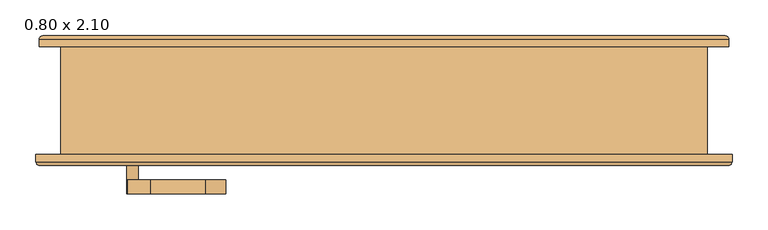
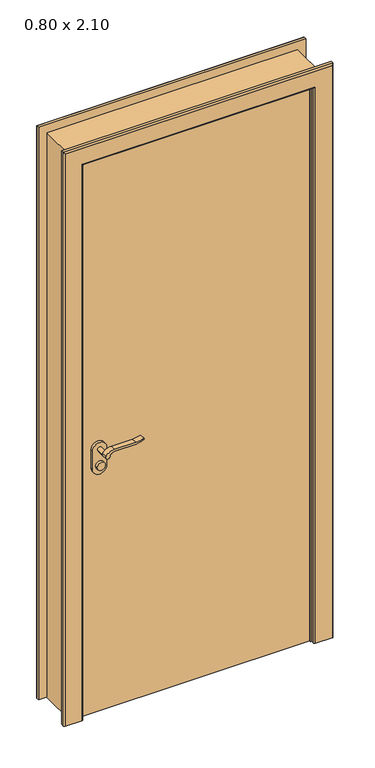
"""IFC4 building model written with IfcOpenShell, lengths in millimetres: door geometry, PORTA_DE_ABRIR_MADEIRA : 0.80 x 2.10."""

import ifcopenshell
import ifcopenshell.guid

model = None  # the IFC model being written
_history = None  # IfcOwnerHistory: only IFC2X3 demands one
_inside = {}  # id of a spatial element -> (the spatial element, [elements in it])
_under = {}  # id of a project, library or spatial element -> (it, [spatial elements below it])
_declared = {}  # id of a project -> (the project, [libraries it declares])
_typed = {}  # id of a type object -> (the type object, [elements of that type])
_made_of = {}  # id of a material, layer set ... -> (it, [elements and type objects made of it])


def new_model(schema):
    """Start an empty IFC model of exactly this schema.

    Asked for "IFC4X3", IfcOpenShell would pick the latest addendum, in which some entities
    have other attributes; the version numbers below select the first issue.
    IFC2X3 requires an IfcOwnerHistory on every rooted entity: one is made here for all.
    """
    global model, _history
    if schema == "IFC4X3":
        model = ifcopenshell.file(schema_version=(4, 3, 0, 0))
    else:
        model = ifcopenshell.file(schema=schema)
    _inside.clear()
    _under.clear()
    _declared.clear()
    _typed.clear()
    _made_of.clear()
    _history = None
    if model.schema == "IFC2X3":
        org = make("IfcOrganization", Name="unknown")
        user = make(
            "IfcPersonAndOrganization",
            ThePerson=make("IfcPerson", FamilyName="unknown"),
            TheOrganization=org,
        )
        app = make(
            "IfcApplication",
            ApplicationDeveloper=org,
            Version="unknown",
            ApplicationFullName="unknown",
            ApplicationIdentifier="unknown",
        )
        _history = make(
            "IfcOwnerHistory",
            OwningUser=user,
            OwningApplication=app,
            ChangeAction="ADDED",
            CreationDate=0,
        )
    return model


def make(cls, **values):
    """One entity of the class cls with the attributes given. An attribute that is None is left unset."""
    return model.create_entity(
        cls, **{name: value for name, value in values.items() if value is not None}
    )


def rooted(cls, **values):
    """An entity with a GlobalId (a new one), such as an element, a storey or a relation."""
    return make(cls, GlobalId=ifcopenshell.guid.new(), OwnerHistory=_history, **values)


def si_unit(unit_type, name, prefix=None):
    """IfcSIUnit, for example si_unit("LENGTHUNIT", "METRE", prefix="MILLI")."""
    return make("IfcSIUnit", UnitType=unit_type, Prefix=prefix, Name=name)


def assignment(units):
    """IfcUnitAssignment: the units of a project."""
    return None if units is None else make("IfcUnitAssignment", Units=units)


def point(xyz):
    """IfcCartesianPoint."""
    return None if xyz is None else make("IfcCartesianPoint", Coordinates=xyz)


def direction(xyz):
    """IfcDirection."""
    return None if xyz is None else make("IfcDirection", DirectionRatios=xyz)


def frame(location, z_axis=None, x_axis=None):
    """IfcAxis2Placement3D, a coordinate frame: its origin and axes. An axis left out is left unset."""
    return make(
        "IfcAxis2Placement3D",
        Location=point(location),
        Axis=direction(z_axis),
        RefDirection=direction(x_axis),
    )


def frame_2d(location, x_axis=None):
    """IfcAxis2Placement2D, a coordinate frame in the plane: its origin and x axis."""
    return make(
        "IfcAxis2Placement2D", Location=point(location), RefDirection=direction(x_axis)
    )


def origin():
    """The frame at (0, 0, 0) with its axes left unset."""
    return frame((0.0, 0.0, 0.0))


def origin_with_axes():
    """The frame at (0, 0, 0) with the z axis (0, 0, 1) and the x axis (1, 0, 0) written out."""
    return frame((0.0, 0.0, 0.0), z_axis=(0.0, 0.0, 1.0), x_axis=(1.0, 0.0, 0.0))


def place(relative_to, where):
    """IfcLocalPlacement: puts the frame where relative to a parent placement (None: the world)."""
    return make(
        "IfcLocalPlacement", PlacementRelTo=relative_to, RelativePlacement=where
    )


def context(
    kind, dimensions, precision=None, world=None, true_north=None, identifier=None
):
    """IfcGeometricRepresentationContext, for example the 3D "Model" context."""
    return make(
        "IfcGeometricRepresentationContext",
        ContextIdentifier=identifier,
        ContextType=kind,
        CoordinateSpaceDimension=dimensions,
        Precision=precision,
        WorldCoordinateSystem=world,
        TrueNorth=true_north,
    )


def project(units=None, contexts=None):
    """IfcProject with its units and contexts."""
    return rooted(
        "IfcProject",
        Name="project",
        RepresentationContexts=contexts,
        UnitsInContext=assignment(units),
    )


def spatial(cls, under=None, at=None, **own):
    """A site, building, storey or space (cls), placed at a placement, below another one or the project."""
    s = rooted(cls, ObjectPlacement=at, **own)
    if under is not None:
        _under.setdefault(under.id(), (under, []))[1].append(s)
    return s


def polyline(points):
    """IfcPolyline through the points."""
    return make("IfcPolyline", Points=[point(p) for p in points])


def circle_curve(where, radius):
    """IfcCircle in the frame where."""
    return make("IfcCircle", Position=where, Radius=radius)


def ellipse_curve(where, semi_axis1, semi_axis2):
    """IfcEllipse in the frame where."""
    return make(
        "IfcEllipse", Position=where, SemiAxis1=semi_axis1, SemiAxis2=semi_axis2
    )


def trimmed(basis, trim1, trim2, sense, master):
    """IfcTrimmedCurve: the piece of a basis curve between two trims."""
    return make(
        "IfcTrimmedCurve",
        BasisCurve=basis,
        Trim1=trim1,
        Trim2=trim2,
        SenseAgreement=sense,
        MasterRepresentation=master,
    )


def segment(curve, same_sense, transition):
    """IfcCompositeCurveSegment."""
    return make(
        "IfcCompositeCurveSegment",
        Transition=transition,
        SameSense=same_sense,
        ParentCurve=curve,
    )


def composite_curve(segments, self_intersect=None):
    """IfcCompositeCurve: segments joined end to end."""
    return make("IfcCompositeCurve", Segments=segments, SelfIntersect=self_intersect)


def outline(outer, holes=None, kind="AREA"):
    """IfcArbitraryClosedProfileDef: a profile drawn as a closed curve; with holes, ...WithVoids."""
    if holes is None:
        return make("IfcArbitraryClosedProfileDef", ProfileType=kind, OuterCurve=outer)
    return make(
        "IfcArbitraryProfileDefWithVoids",
        ProfileType=kind,
        OuterCurve=outer,
        InnerCurves=holes,
    )


def extrude(swept, where, along, depth):
    """IfcExtrudedAreaSolid: the profile swept, set in the frame where, extruded along a direction by depth."""
    return make(
        "IfcExtrudedAreaSolid",
        SweptArea=swept,
        Position=where,
        ExtrudedDirection=direction(along),
        Depth=depth,
    )


def faces_of(points, faces, orient=None, outer=None):
    """IfcFace entities. A face is a list of loops; a loop is a list of indices into points, from 0.

    orient and outer hold one flag for each loop. By default every Orientation is true, the
    first loop of a face is its IfcFaceOuterBound and the others are IfcFaceBound.
    """
    made = []
    for i, loops in enumerate(faces):
        bounds = []
        for j, loop in enumerate(loops):
            is_outer = j == 0 if outer is None else outer[i][j]
            bounds.append(
                make(
                    "IfcFaceOuterBound" if is_outer else "IfcFaceBound",
                    Bound=make("IfcPolyLoop", Polygon=[points[k] for k in loop]),
                    Orientation=True if orient is None else orient[i][j],
                )
            )
        made.append(make("IfcFace", Bounds=bounds))
    return made


def faceted_brep(points, faces, orient=None, outer=None, voids=None):
    """IfcFacetedBrep: a solid bounded by flat faces; with voids (closed shells), ...WithVoids."""
    shared = [point(p) for p in points]
    hull = make("IfcClosedShell", CfsFaces=faces_of(shared, faces, orient, outer))
    if voids is None:
        return make("IfcFacetedBrep", Outer=hull)
    return make(
        "IfcFacetedBrepWithVoids",
        Outer=hull,
        Voids=[
            make(cls, CfsFaces=faces_of(shared, fs, o, b)) for cls, fs, o, b in voids
        ],
    )


def shape(context_of_items, identifier, shape_type, items):
    """IfcShapeRepresentation: the items that make up one representation, for example the "Body"."""
    return make(
        "IfcShapeRepresentation",
        ContextOfItems=context_of_items,
        RepresentationIdentifier=identifier,
        RepresentationType=shape_type,
        Items=items,
    )


def source(mapping_origin, context_of_items, identifier, shape_type, items):
    """IfcRepresentationMap: a shape defined once, which mapped items show again and again."""
    return make(
        "IfcRepresentationMap",
        MappingOrigin=mapping_origin,
        MappedRepresentation=shape(context_of_items, identifier, shape_type, items),
    )


def transform(
    local_origin,
    x_axis=None,
    y_axis=None,
    z_axis=None,
    scale=None,
    scale2=None,
    scale3=None,
    uniform=True,
):
    """IfcCartesianTransformationOperator3D, or its non-uniform kind. x_axis, y_axis, z_axis: its Axis1, 2, 3."""
    if uniform:
        return make(
            "IfcCartesianTransformationOperator3D",
            Axis1=direction(x_axis),
            Axis2=direction(y_axis),
            LocalOrigin=point(local_origin),
            Scale=scale,
            Axis3=direction(z_axis),
        )
    return make(
        "IfcCartesianTransformationOperator3DnonUniform",
        Axis1=direction(x_axis),
        Axis2=direction(y_axis),
        LocalOrigin=point(local_origin),
        Scale=scale,
        Axis3=direction(z_axis),
        Scale2=scale2,
        Scale3=scale3,
    )


def mapped(mapping_source, mapping_target):
    """IfcMappedItem: shows the shape of a source again, moved by a transform."""
    return make(
        "IfcMappedItem", MappingSource=mapping_source, MappingTarget=mapping_target
    )


def made_of(thing, what):
    """Note that an element or type object is made of a material, layer set ...; save() writes the relation."""
    if what is not None:
        _made_of.setdefault(what.id(), (what, []))[1].append(thing)
    return thing


def element(
    cls,
    number,
    at=None,
    inside=None,
    cuts=None,
    type_object=None,
    material=None,
    context=None,
    identifier="Body",
    shape_type=None,
    held_by="IfcProductDefinitionShape",
    body=None,
    shapes=None,
    **own,
):
    """One element of the class cls, such as IfcWall. Its Tag is "e" and its number.

    at: its placement. inside: the storey or other place that contains it. cuts: it is an
    opening in that element (IfcRelVoidsElement). A single representation is given by context,
    identifier, shape_type and body (its items); several are given by shapes. held_by: the class
    of the entity that holds the representations. save() writes the other relations.
    """
    e = rooted(cls, Tag="e%d" % number, ObjectPlacement=at, **own)
    if body is not None:
        shapes = [shape(context, identifier, shape_type, body)]
    if shapes is not None:
        e.Representation = make(held_by, Representations=shapes)
    if inside is not None:
        _inside.setdefault(inside.id(), (inside, []))[1].append(e)
    if cuts is not None:
        rooted(
            "IfcRelVoidsElement", RelatingBuildingElement=cuts, RelatedOpeningElement=e
        )
    if type_object is not None:
        _typed.setdefault(type_object.id(), (type_object, []))[1].append(e)
    return made_of(e, material)


def aggregate(whole, parts):
    """IfcRelAggregates: a whole, such as a stair, and the parts it consists of."""
    return rooted("IfcRelAggregates", RelatingObject=whole, RelatedObjects=parts)


def save(model, path):
    """Write the relations noted so far, then the file.

    IfcRelAggregates (storeys below a building ...), IfcRelContainedInSpatialStructure (elements
    in a storey), IfcRelDefinesByType, IfcRelAssociatesMaterial and IfcRelDeclares: one each for
    every whole, place, type object, material and project.
    """
    for whole, parts in _under.values():
        aggregate(whole, parts)
    for where, things in _inside.values():
        rooted(
            "IfcRelContainedInSpatialStructure",
            RelatedElements=things,
            RelatingStructure=where,
        )
    for kind, things in _typed.values():
        rooted("IfcRelDefinesByType", RelatedObjects=things, RelatingType=kind)
    for what, things in _made_of.values():
        rooted("IfcRelAssociatesMaterial", RelatedObjects=things, RelatingMaterial=what)
    for by, libraries in _declared.values():
        rooted("IfcRelDeclares", RelatingContext=by, RelatedDefinitions=libraries)
    model.write(path)


def plane_surface(at):
    """IfcPlane: the flat surface through the origin of the frame at, square to its z axis."""
    return make("IfcPlane", Position=at)


def cylinder_surface(at, radius):
    """IfcCylindricalSurface: all points at the distance radius from the z axis of the frame at."""
    return make("IfcCylindricalSurface", Position=at, Radius=radius)


def advanced_brep(points, edges, surfaces, faces):
    """IfcAdvancedBrep: a solid bounded by faces that lie on surfaces and meet in shared edges.

    An edge is (start, end): straight between two places in points (the first is 0);
    or (start, end, curve); or (start, end, curve, False) where it runs against its curve.
    A face is (place in surfaces, loops), or (place, loops, False) where it looks against
    its surface's normal. A loop lists edges by number (the first is 1), with a minus sign
    where the edge is run from its end to its start. The first loop is the outer one.
    """
    corners = [point(p) for p in points]
    vertices = [make("IfcVertexPoint", VertexGeometry=c) for c in corners]
    made = []
    for start, end, *more in edges:
        made.append(
            make(
                "IfcEdgeCurve",
                EdgeStart=vertices[start],
                EdgeEnd=vertices[end],
                EdgeGeometry=more[0] if more else make("IfcPolyline", Points=[corners[start], corners[end]]),
                SameSense=more[1] if len(more) > 1 else True,
            )
        )
    hull = []
    for where, loops, *sense in faces:
        bounds = []
        for j, loop in enumerate(loops):
            ring = [make("IfcOrientedEdge", EdgeElement=made[abs(k) - 1], Orientation=k > 0) for k in loop]
            bounds.append(
                make(
                    "IfcFaceOuterBound" if j == 0 else "IfcFaceBound",
                    Bound=make("IfcEdgeLoop", EdgeList=ring),
                    Orientation=True,
                )
            )
        hull.append(make("IfcAdvancedFace", Bounds=bounds, FaceSurface=surfaces[where], SameSense=sense[0] if sense else True))
    return make("IfcAdvancedBrep", Outer=make("IfcClosedShell", CfsFaces=hull))


def door_0_80_x_2_10_69306b0e(model_context):
    return source(origin(), model_context, "Body", "SolidModel", [
        extrude(outline(composite_curve([segment(trimmed(circle_curve(frame_2d((940.0, -350.0)), 15.0), [point((940.0, -335.0))], [point((940.0, -365.0))], False, "CARTESIAN"), True, "CONTINUOUS"), segment(trimmed(circle_curve(frame_2d((940.0, -350.0)), 15.0), [point((940.0, -365.0))], [point((940.0, -335.0))], False, "CARTESIAN"), True, "CONTINUOUS")], self_intersect=False)), frame((0.0, -25.0, 0.0), z_axis=(0.0, 1.0, 0.0), x_axis=(0.0, 0.0, 1.0)), (0.0, 0.0, 1.0), 10.0),
        extrude(outline(composite_curve([segment(trimmed(circle_curve(frame_2d((940.0, -350.0)), 15.0), [point((940.0, -335.0))], [point((940.0, -365.0))], False, "CARTESIAN"), True, "CONTINUOUS"), segment(trimmed(circle_curve(frame_2d((940.0, -350.0)), 15.0), [point((940.0, -365.0))], [point((940.0, -335.0))], False, "CARTESIAN"), True, "CONTINUOUS")], self_intersect=False)), frame((0.0, -90.0, 0.0), z_axis=(0.0, 1.0, 0.0), x_axis=(0.0, 0.0, 1.0)), (0.0, 0.0, 1.0), 10.0),
        extrude(outline(composite_curve([segment(trimmed(circle_curve(frame_2d((1000.0, -350.0)), 8.0), [point((1004.6523287, -356.5081363))], [point((1000.0, -342.0))], False, "CARTESIAN"), True, "CONTINUOUS"), segment(trimmed(circle_curve(frame_2d((994.8738613, -324.6138099)), 18.1261387), [point((1000.0, -342.0))], [point((1013.0, -324.6138099))], True, "CARTESIAN"), True, "CONTINUOUS"), segment(polyline([(1013.0, -324.6138099), (1013.0, -248.3564091)]), True, "CONTINUOUS"), segment(trimmed(circle_curve(frame_2d((1072.2709207, -251.9396612)), 59.3791355), [point((1013.0, -248.3564091))], [point((1022.2135558, -220.0))], False, "CARTESIAN"), True, "CONTINUOUS"), segment(polyline([(1022.2135558, -220.0), (1025.0, -220.0)]), True, "CONTINUOUS"), segment(trimmed(circle_curve(frame_2d((1103.2850638, -248.4227909)), 83.2850902), [point((1025.0, -220.0))], [point((1020.0, -248.3564091))], True, "CARTESIAN"), True, "CONTINUOUS"), segment(polyline([(1020.0, -248.3564091), (1020.0, -324.6325667)]), True, "CONTINUOUS"), segment(trimmed(circle_curve(frame_2d((982.7555521, -326.3324871)), 37.2832219), [point((1020.0, -324.6325667))], [point((1004.6523287, -356.5081363))], False, "CARTESIAN"), True, "CONTINUOUS")], self_intersect=False)), frame((0.0, 5.0, 0.0), z_axis=(0.0, 1.0, 0.0), x_axis=(0.0, 0.0, 1.0)), (0.0, 0.0, 1.0), 20.0),
        extrude(outline(composite_curve([segment(trimmed(circle_curve(frame_2d((994.8738682, -324.6138122)), 18.1261318), [point((999.9999903, -342.0))], [point((1013.0, -324.6138122))], True, "CARTESIAN"), True, "CONTINUOUS"), segment(polyline([(1013.0, -324.6138122), (1013.0, -248.3564091)]), True, "CONTINUOUS"), segment(trimmed(circle_curve(frame_2d((1072.2709207, -251.9396612)), 59.3791355), [point((1013.0, -248.3564091))], [point((1022.2135558, -220.0))], False, "CARTESIAN"), True, "CONTINUOUS"), segment(polyline([(1022.2135558, -220.0), (1025.0, -220.0)]), True, "CONTINUOUS"), segment(trimmed(circle_curve(frame_2d((1103.2850638, -248.4227909)), 83.2850902), [point((1025.0, -220.0))], [point((1020.0, -248.3564091))], True, "CARTESIAN"), True, "CONTINUOUS"), segment(polyline([(1020.0, -248.3564091), (1020.0, -324.6325667)]), True, "CONTINUOUS"), segment(trimmed(circle_curve(frame_2d((982.7555521, -326.3324871)), 37.2832219), [point((1020.0, -324.6325667))], [point((1004.6523287, -356.5081363))], False, "CARTESIAN"), True, "CONTINUOUS"), segment(trimmed(circle_curve(frame_2d((1000.0, -350.0)), 8.0), [point((1004.6523287, -356.5081363))], [point((999.9999903, -342.0))], False, "CARTESIAN"), True, "CONTINUOUS")], self_intersect=False)), frame((0.0, -130.0, 0.0), z_axis=(0.0, 1.0, 0.0), x_axis=(0.0, 0.0, 1.0)), (0.0, 0.0, 1.0), 20.0),
        extrude(outline(composite_curve([segment(trimmed(circle_curve(frame_2d((1000.0, -350.0)), 8.0), [point((1000.0, -342.0))], [point((1000.0, -358.0))], False, "CARTESIAN"), True, "CONTINUOUS"), segment(trimmed(circle_curve(frame_2d((1000.0, -350.0)), 8.0), [point((1000.0, -358.0))], [point((1000.0, -342.0))], False, "CARTESIAN"), True, "CONTINUOUS")], self_intersect=False)), frame((0.0, -25.0, 0.0), z_axis=(0.0, 1.0, 0.0), x_axis=(0.0, 0.0, 1.0)), (0.0, 0.0, 1.0), 30.0),
        extrude(outline(composite_curve([segment(trimmed(circle_curve(frame_2d((1000.0, -350.0)), 8.0), [point((1000.0, -342.0))], [point((1000.0, -358.0))], False, "CARTESIAN"), True, "CONTINUOUS"), segment(trimmed(circle_curve(frame_2d((1000.0, -350.0)), 8.0), [point((1000.0, -358.0))], [point((1000.0, -342.0))], False, "CARTESIAN"), True, "CONTINUOUS")], self_intersect=False)), frame((0.0, -110.0, 0.0), z_axis=(0.0, 1.0, 0.0), x_axis=(0.0, 0.0, 1.0)), (0.0, 0.0, 1.0), 30.0),
        extrude(outline(composite_curve([segment(trimmed(circle_curve(frame_2d((930.0, -350.0)), 25.0), [point((930.0, -375.0))], [point((930.0, -325.0))], False, "CARTESIAN"), True, "CONTINUOUS"), segment(polyline([(930.0, -325.0), (1000.0, -325.0)]), True, "CONTINUOUS"), segment(trimmed(circle_curve(frame_2d((1000.0, -350.0)), 25.0), [point((1000.0, -325.0))], [point((1000.0, -375.0))], False, "CARTESIAN"), True, "CONTINUOUS"), segment(polyline([(1000.0, -375.0), (930.0, -375.0)]), True, "CONTINUOUS")], self_intersect=False)), frame((0.0, -35.0, 0.0), z_axis=(0.0, 1.0, 0.0), x_axis=(0.0, 0.0, 1.0)), (0.0, 0.0, 1.0), 10.0),
        extrude(outline(composite_curve([segment(trimmed(circle_curve(frame_2d((930.0, -350.0)), 25.0), [point((930.0, -375.0))], [point((930.0, -325.0))], False, "CARTESIAN"), True, "CONTINUOUS"), segment(polyline([(930.0, -325.0), (1000.0, -325.0)]), True, "CONTINUOUS"), segment(trimmed(circle_curve(frame_2d((1000.0, -350.0)), 25.0), [point((1000.0, -325.0))], [point((1000.0, -375.0))], False, "CARTESIAN"), True, "CONTINUOUS"), segment(polyline([(1000.0, -375.0), (930.0, -375.0)]), True, "CONTINUOUS")], self_intersect=False)), frame((0.0, -80.0, 0.0), z_axis=(0.0, 1.0, 0.0), x_axis=(0.0, 0.0, 1.0)), (0.0, 0.0, 1.0), 10.0),
        faceted_brep([(-410.0, -35.0, 0.0), (-410.0, -75.0, 0.0), (-450.0, -75.0, 0.0), (-450.0, 75.0, 0.0), (-400.0, 75.0, 0.0), (-400.0, -35.0, 0.0), (-410.0, -35.0, 2100.0), (-410.0, -75.0, 2100.0), (410.0, -75.0, 2100.0), (410.0, -75.0, 0.0), (450.0, -75.0, 0.0), (450.0, -75.0, 2140.0), (-450.0, -75.0, 2140.0), (-450.0, 75.0, 2140.0), (450.0, 75.0, 2140.0), (450.0, 75.0, 0.0), (400.0, 75.0, 0.0), (400.0, 75.0, 2090.0), (-400.0, 75.0, 2090.0), (-400.0, -35.0, 2090.0), (400.0, -35.0, 2090.0), (400.0, -35.0, 0.0), (410.0, -35.0, 0.0), (410.0, -35.0, 2100.0)], [[[0, 1, 2, 3, 4, 5]], [[1, 0, 6, 7]], [[2, 1, 7, 8, 9, 10, 11, 12]], [[3, 2, 12, 13]], [[4, 3, 13, 14, 15, 16, 17, 18]], [[5, 4, 18, 19]], [[0, 5, 19, 20, 21, 22, 23, 6]], [[20, 17, 16, 21]], [[22, 21, 16, 15, 10, 9]], [[8, 23, 22, 9]], [[14, 11, 10, 15]], [[13, 12, 11, 14]], [[19, 18, 17, 20]], [[7, 6, 23, 8]]]),
        advanced_brep(
        [(-480.0, 75.3, 0.0), (-480.0, 85.3, 0.0), (-475.0, 90.3, 0.0), (-415.0, 90.3, 0.0), (-410.0, 85.3, 0.0), (-410.0, 75.3, 0.0), (-480.0, 75.3, 2170.0), (-480.0, 85.3, 2170.0), (-475.0, 90.3, 2165.0), (475.0, 90.3, 2165.0), (475.0, 90.3, 0.0), (415.0, 90.3, 0.0), (415.0, 90.3, 2105.0), (-415.0, 90.3, 2105.0), (-410.0, 85.3, 2100.0), (-410.0, 75.3, 2100.0), (410.0, 75.3, 2100.0), (410.0, 75.3, 0.0), (480.0, 75.3, 0.0), (480.0, 75.3, 2170.0), (410.0, 85.3, 0.0), (480.0, 85.3, 0.0), (410.0, 85.3, 2100.0), (480.0, 85.3, 2170.0)],
        [
            (0, 1),
            (1, 2, circle_curve(frame((-475.0, 85.3, 0.0), z_axis=(0.0, 0.0, -1.0), x_axis=(-1.0, 0.0, 0.0)), 5.0)),
            (2, 3),
            (3, 4, circle_curve(frame((-415.0, 85.3, 0.0), z_axis=(0.0, 0.0, -1.0), x_axis=(-1.0, 0.0, 0.0)), 5.0)),
            (4, 5),
            (5, 0),
            (0, 6),
            (6, 7),
            (7, 1),
            (7, 8, ellipse_curve(frame((-475.0, 85.3, 2165.0), z_axis=(-0.7071067811865475, 0.0, -0.7071067811865475), x_axis=(0.7071067811865474, 0.0, -0.7071067811865476)), 7.0710678, 5.0)),
            (8, 2),
            (8, 9),
            (9, 10),
            (10, 11),
            (11, 12),
            (12, 13),
            (13, 3),
            (13, 14, ellipse_curve(frame((-415.0, 85.3, 2105.0), z_axis=(-0.7071067811865475, 0.0, -0.7071067811865475), x_axis=(0.7071067811865474, 0.0, -0.7071067811865476)), 7.0710678, 5.0)),
            (14, 4),
            (14, 15),
            (15, 5),
            (15, 16),
            (16, 17),
            (17, 18),
            (18, 19),
            (19, 6),
            (17, 20),
            (20, 11, circle_curve(frame((415.0, 85.3, 0.0), z_axis=(0.0, 0.0, -1.0), x_axis=(1.0, 0.0, 0.0)), 5.0)),
            (10, 21, circle_curve(frame((475.0, 85.3, 0.0), z_axis=(0.0, 0.0, -1.0), x_axis=(1.0, 0.0, 0.0)), 5.0)),
            (21, 18),
            (16, 22),
            (22, 20),
            (22, 12, ellipse_curve(frame((415.0, 85.3, 2105.0), z_axis=(0.7071067811865475, 0.0, -0.7071067811865475), x_axis=(0.7071067811865474, 0.0, 0.7071067811865476)), 7.0710678, 5.0)),
            (9, 23, ellipse_curve(frame((475.0, 85.3, 2165.0), z_axis=(0.7071067811865475, 0.0, -0.7071067811865475), x_axis=(0.7071067811865474, 0.0, 0.7071067811865476)), 7.0710678, 5.0)),
            (23, 21),
            (23, 19),
            (23, 7),
            (14, 22),
        ],
        [
            plane_surface(frame((-450.0, -75.0, 0.0), z_axis=(0.0, 0.0, -1.0), x_axis=(0.0, -1.0, 0.0))),
            plane_surface(frame((-480.0, 75.3, 0.0), z_axis=(-1.0, 0.0, 0.0), x_axis=(0.0, 0.0, 1.0))),
            cylinder_surface(frame((-475.0, 85.3, 0.0), z_axis=(0.0, 0.0, -1.0), x_axis=(-1.0, 0.0, 0.0)), 5.0),
            plane_surface(frame((-475.0, 90.3, 0.0), z_axis=(0.0, 1.0, 0.0), x_axis=(0.0, 0.0, 1.0))),
            cylinder_surface(frame((-415.0, 85.3, 0.0), z_axis=(0.0, 0.0, -1.0), x_axis=(-1.0, 0.0, 0.0)), 5.0),
            plane_surface(frame((-410.0, 85.3, 0.0), z_axis=(1.0, 0.0, 0.0), x_axis=(0.0, 0.0, 1.0))),
            plane_surface(frame((-410.0, 75.3, 0.0), z_axis=(0.0, -1.0, 0.0), x_axis=(0.0, 0.0, 1.0))),
            plane_surface(frame((450.0, -75.0, 0.0), z_axis=(0.0, 0.0, -1.0), x_axis=(0.0, -1.0, 0.0))),
            plane_surface(frame((410.0, 85.3, 2100.0), z_axis=(-1.0, 0.0, 0.0), x_axis=(0.0, 0.0, -1.0))),
            cylinder_surface(frame((415.0, 85.3, 2140.0), z_axis=(0.0, 0.0, 1.0), x_axis=(1.0, 0.0, 0.0)), 5.0),
            cylinder_surface(frame((475.0, 85.3, 2140.0), z_axis=(0.0, 0.0, 1.0), x_axis=(1.0, 0.0, 0.0)), 5.0),
            plane_surface(frame((480.0, 75.3, 2170.0), z_axis=(1.0, 0.0, 0.0), x_axis=(0.0, 0.0, -1.0))),
            plane_surface(frame((-480.0, 75.3, 2170.0), z_axis=(0.0, 0.0, 1.0), x_axis=(1.0, 0.0, 0.0))),
            plane_surface(frame((-410.0, 85.3, 2100.0), z_axis=(0.0, 0.0, -1.0), x_axis=(1.0, 0.0, 0.0))),
            cylinder_surface(frame((-450.0, 85.3, 2165.0), z_axis=(-1.0, 0.0, 0.0), x_axis=(0.0, 0.0, 1.0)), 5.0),
            cylinder_surface(frame((-450.0, 85.3, 2105.0), z_axis=(-1.0, 0.0, 0.0), x_axis=(0.0, 0.0, 1.0)), 5.0),
        ],
        [
            (0, [[1, 2, 3, 4, 5, 6]]),
            (1, [[-1, 7, 8, 9]]),
            (2, [[-2, -9, 10, 11]]),
            (3, [[-3, -11, 12, 13, 14, 15, 16, 17]]),
            (4, [[-4, -17, 18, 19]]),
            (5, [[-5, -19, 20, 21]]),
            (6, [[-6, -21, 22, 23, 24, 25, 26, -7]]),
            (7, [[-24, 27, 28, -14, 29, 30]]),
            (8, [[31, 32, -27, -23]]),
            (9, [[33, -15, -28, -32]]),
            (10, [[34, 35, -29, -13]]),
            (11, [[36, -25, -30, -35]]),
            (12, [[-8, -26, -36, 37]]),
            (13, [[-20, 38, -31, -22]]),
            (14, [[-10, -37, -34, -12]]),
            (15, [[-18, -16, -33, -38]]),
        ],
    ),
        advanced_brep(
        [(-479.3155593, -90.2647517, 0.0), (-484.3155593, -85.2647517, 0.0), (-484.3155593, -75.2647517, 0.0), (-414.3155593, -75.2647517, 0.0), (-414.3155593, -85.2647517, 0.0), (-419.3155593, -90.2647517, 0.0), (-479.3155593, -90.2647517, 2169.3155593), (-484.3155593, -85.2647517, 2174.3155593), (-484.3155593, -75.2647517, 2174.3155593), (484.3155593, -75.2647517, 2174.3155593), (484.3155593, -75.2647517, 0.0), (414.3155593, -75.2647517, 0.0), (414.3155593, -75.2647517, 2104.3155593), (-414.3155593, -75.2647517, 2104.3155593), (-414.3155593, -85.2647517, 2104.3155593), (-419.3155593, -90.2647517, 2109.3155593), (419.3155593, -90.2647517, 2109.3155593), (419.3155593, -90.2647517, 0.0), (479.3155593, -90.2647517, 0.0), (479.3155593, -90.2647517, 2169.3155593), (414.3155593, -85.2647517, 0.0), (484.3155593, -85.2647517, 0.0), (414.3155593, -85.2647517, 2104.3155593), (484.3155593, -85.2647517, 2174.3155593)],
        [
            (0, 1, circle_curve(frame((-479.3155593, -85.2647517, 0.0), z_axis=(0.0, 0.0, -1.0), x_axis=(-1.0, 0.0, 0.0)), 5.0)),
            (1, 2),
            (2, 3),
            (3, 4),
            (4, 5, circle_curve(frame((-419.3155593, -85.2647517, 0.0), z_axis=(0.0, 0.0, -1.0), x_axis=(-1.0, 0.0, 0.0)), 5.0)),
            (5, 0),
            (0, 6),
            (6, 7, ellipse_curve(frame((-479.3155593, -85.2647517, 2169.3155593), z_axis=(-0.7071067811865475, 0.0, -0.7071067811865475), x_axis=(0.7071067811865474, 0.0, -0.7071067811865476)), 7.0710678, 5.0)),
            (7, 1),
            (7, 8),
            (8, 2),
            (8, 9),
            (9, 10),
            (10, 11),
            (11, 12),
            (12, 13),
            (13, 3),
            (13, 14),
            (14, 4),
            (14, 15, ellipse_curve(frame((-419.3155593, -85.2647517, 2109.3155593), z_axis=(-0.7071067811865475, 0.0, -0.7071067811865475), x_axis=(0.7071067811865474, 0.0, -0.7071067811865476)), 7.0710678, 5.0)),
            (15, 5),
            (15, 16),
            (16, 17),
            (17, 18),
            (18, 19),
            (19, 6),
            (17, 20, circle_curve(frame((419.3155593, -85.2647517, 0.0), z_axis=(0.0, 0.0, -1.0), x_axis=(1.0, 0.0, 0.0)), 5.0)),
            (20, 11),
            (10, 21),
            (21, 18, circle_curve(frame((479.3155593, -85.2647517, 0.0), z_axis=(0.0, 0.0, -1.0), x_axis=(1.0, 0.0, 0.0)), 5.0)),
            (16, 22, ellipse_curve(frame((419.3155593, -85.2647517, 2109.3155593), z_axis=(0.7071067811865475, 0.0, -0.7071067811865475), x_axis=(0.7071067811865474, 0.0, 0.7071067811865476)), 7.0710678, 5.0)),
            (22, 20),
            (22, 12),
            (9, 23),
            (23, 21),
            (23, 19, ellipse_curve(frame((479.3155593, -85.2647517, 2169.3155593), z_axis=(0.7071067811865475, 0.0, -0.7071067811865475), x_axis=(0.7071067811865474, 0.0, 0.7071067811865476)), 7.0710678, 5.0)),
            (7, 23),
            (22, 14),
        ],
        [
            plane_surface(frame((-450.0, -75.0, 0.0), z_axis=(0.0, 0.0, -1.0), x_axis=(0.0, -1.0, 0.0))),
            cylinder_surface(frame((-479.3155593, -85.2647517, 0.0), z_axis=(0.0, 0.0, -1.0), x_axis=(-1.0, 0.0, 0.0)), 5.0),
            plane_surface(frame((-484.3155593, -85.2647517, 0.0), z_axis=(-1.0, 0.0, 0.0), x_axis=(0.0, 0.0, 1.0))),
            plane_surface(frame((-484.3155593, -75.2647517, 0.0), z_axis=(0.0, 1.0, 0.0), x_axis=(0.0, 0.0, 1.0))),
            plane_surface(frame((-414.3155593, -75.2647517, 0.0), z_axis=(1.0, 0.0, 0.0), x_axis=(0.0, 0.0, 1.0))),
            cylinder_surface(frame((-419.3155593, -85.2647517, 0.0), z_axis=(0.0, 0.0, -1.0), x_axis=(-1.0, 0.0, 0.0)), 5.0),
            plane_surface(frame((-419.3155593, -90.2647517, 0.0), z_axis=(0.0, -1.0, 0.0), x_axis=(0.0, 0.0, 1.0))),
            plane_surface(frame((450.0, -75.0, 0.0), z_axis=(0.0, 0.0, -1.0), x_axis=(0.0, -1.0, 0.0))),
            cylinder_surface(frame((419.3155593, -85.2647517, 2140.0), z_axis=(0.0, 0.0, 1.0), x_axis=(1.0, 0.0, 0.0)), 5.0),
            plane_surface(frame((414.3155593, -75.2647517, 2104.3155593), z_axis=(-1.0, 0.0, 0.0), x_axis=(0.0, 0.0, -1.0))),
            plane_surface(frame((484.3155593, -85.2647517, 2174.3155593), z_axis=(1.0, 0.0, 0.0), x_axis=(0.0, 0.0, -1.0))),
            cylinder_surface(frame((479.3155593, -85.2647517, 2140.0), z_axis=(0.0, 0.0, 1.0), x_axis=(1.0, 0.0, 0.0)), 5.0),
            plane_surface(frame((-484.3155593, -85.2647517, 2174.3155593), z_axis=(0.0, 0.0, 1.0), x_axis=(1.0, 0.0, 0.0))),
            plane_surface(frame((-414.3155593, -75.2647517, 2104.3155593), z_axis=(0.0, 0.0, -1.0), x_axis=(1.0, 0.0, 0.0))),
            cylinder_surface(frame((-450.0, -85.2647517, 2169.3155593), z_axis=(-1.0, 0.0, 0.0), x_axis=(0.0, 0.0, 1.0)), 5.0),
            cylinder_surface(frame((-450.0, -85.2647517, 2109.3155593), z_axis=(-1.0, 0.0, 0.0), x_axis=(0.0, 0.0, 1.0)), 5.0),
        ],
        [
            (0, [[1, 2, 3, 4, 5, 6]]),
            (1, [[-1, 7, 8, 9]]),
            (2, [[-2, -9, 10, 11]]),
            (3, [[-3, -11, 12, 13, 14, 15, 16, 17]]),
            (4, [[-4, -17, 18, 19]]),
            (5, [[-5, -19, 20, 21]]),
            (6, [[-6, -21, 22, 23, 24, 25, 26, -7]]),
            (7, [[-24, 27, 28, -14, 29, 30]]),
            (8, [[31, 32, -27, -23]]),
            (9, [[33, -15, -28, -32]]),
            (10, [[34, 35, -29, -13]]),
            (11, [[36, -25, -30, -35]]),
            (12, [[-10, 37, -34, -12]]),
            (13, [[-18, -16, -33, 38]]),
            (14, [[-8, -26, -36, -37]]),
            (15, [[-20, -38, -31, -22]]),
        ],
    ),
        extrude(outline(polyline([(410.0, -70.0), (-410.0, -70.0), (-410.0, -35.0), (410.0, -35.0), (410.0, -70.0)])), origin_with_axes(), (0.0, 0.0, 1.0), 2100.0),
    ])


if __name__ == "__main__":
    model = new_model("IFC4")
    model_context = context("Model", 3, world=origin())
    ifc_project = project(units=[si_unit("LENGTHUNIT", "METRE", prefix="MILLI")], contexts=[model_context])
    site = spatial("IfcSite", under=ifc_project)
    building = spatial("IfcBuilding", under=site)
    placement = place(None, origin())
    door_0_80_x_2_10_shape = door_0_80_x_2_10_69306b0e(model_context)
    element("IfcDoor", 1, ObjectType="PORTA_DE_ABRIR_MADEIRA : 0.80 x 2.10", at=placement, inside=building, context=model_context, shape_type="MappedRepresentation", body=[
        mapped(door_0_80_x_2_10_shape, transform((0.0, 0.0, 0.0), x_axis=(1.0, 0.0, 0.0), y_axis=(0.0, 1.0, 0.0), z_axis=(0.0, 0.0, 1.0))),
    ])
    save(model, "model.ifc")

# Revit data of these elements
# Type "PORTA_DE_ABRIR_MADEIRA : 0.80 x 2.10"
#   Type Mark = "P2"
#   Analytic Construction = "<Nenhum>"
#   Rough Width = 0.90 m
#   Projeção da estrutura externa = 0.50 m
#   Projeção da estrutura interna = 0.025 m
#   Largura da estrutura = 0.075 m
#   Rough Height = 2.15 m
#   Height = 2.10 m
#   Width = 0.80 m
#   Soleira [instance default] = no
#   Material do batente = .BATENTE E GUARNIÇÃO
#   Material da maçaneta = .AÇO INOXIDÁVEL ESCOVADO
#   Material da folha da porta = .FOLHA DA PORTA
#   Material da Soleira [instance default] = none
#   Function = (empty or 0)
#   Wall Closure = (empty or 0)
# Element 1 (IfcDoor, "PORTA_DE_ABRIR_MADEIRA : 0.80 x 2.10")
#   Materials on its faces: ".AÇO INOXIDÁVEL ESCOVADO", ".BATENTE E GUARNIÇÃO", ".FOLHA DA PORTA"
# Materials
#   ".BATENTE E GUARNIÇÃO": class "Madeira", colour RGB 215 186 156, transparency 0, Cost = 0
#   ".AÇO INOXIDÁVEL ESCOVADO": class "Metal", colour RGB 189 187 185, transparency 0, Description = "Stainless Steel 18/8, brushed finish", Cost = 0
#   ".FOLHA DA PORTA": class "Madeira", colour RGB 148 119 91, transparency 0, Cost = 0
